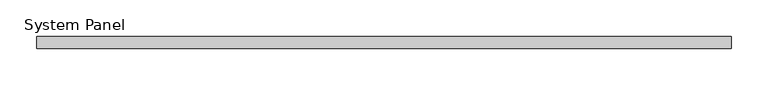
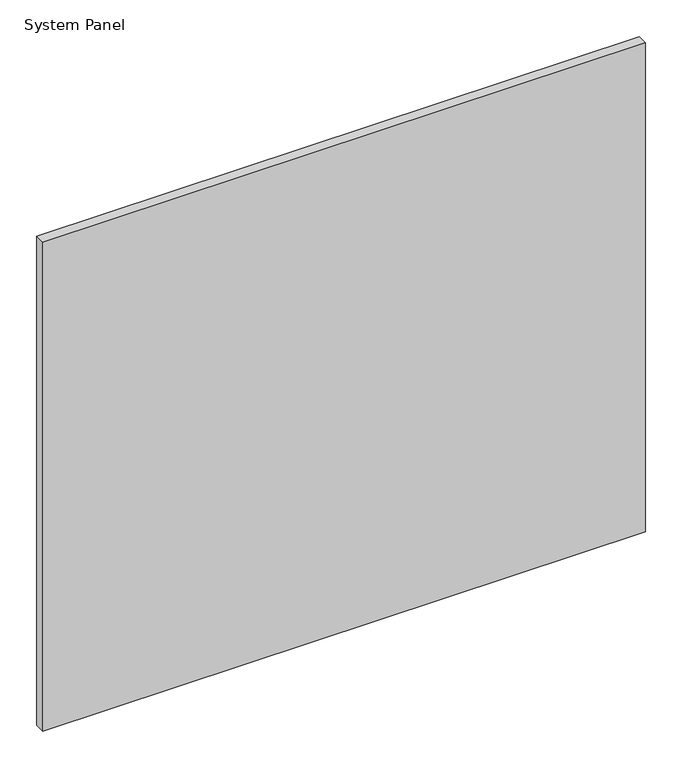
"""IFC4 building model written with IfcOpenShell, lengths in millimetres: plate geometry, System Panel : 로이복층유리_16."""

from ifc_helpers import new_model, si_unit, origin, origin_with_axes, place, context, project, spatial, polyline, outline, extrude, source, transform, mapped, element, save


def system_panel_04b33422(model_context):
    return source(origin(), model_context, "Body", "SweptSolid", [
        extrude(outline(polyline([(472.5, -8.0), (-472.5, -8.0), (-472.5, 8.0), (472.5, 8.0), (472.5, -8.0)])), origin_with_axes(), (0.0, 0.0, 1.0), 810.0),
    ])


if __name__ == "__main__":
    model = new_model("IFC4")
    model_context = context("Model", 3, world=origin())
    ifc_project = project(units=[si_unit("LENGTHUNIT", "METRE", prefix="MILLI")], contexts=[model_context])
    site = spatial("IfcSite", under=ifc_project)
    building = spatial("IfcBuilding", under=site)
    placement = place(None, origin())
    system_panel_shape = system_panel_04b33422(model_context)
    element("IfcPlate", 1, ObjectType="System Panel : 로이복층유리_16", at=placement, inside=building, context=model_context, shape_type="MappedRepresentation", body=[
        mapped(system_panel_shape, transform((0.0, 0.0, 0.0), x_axis=(1.0, 0.0, 0.0), y_axis=(0.0, 1.0, 0.0), z_axis=(0.0, 0.0, 1.0))),
    ])
    save(model, "model.ifc")

# Revit data of these elements
# Element 1 (IfcPlate, "System Panel : 로이복층유리_16")
#   Materials on its faces: "00_Glass_Glass"
# Materials
#   "00_Glass_Glass": class "Glass", colour RGB 218 227 224, transparency 0.85, Description = "Glass", Cost = 0, Image = none
